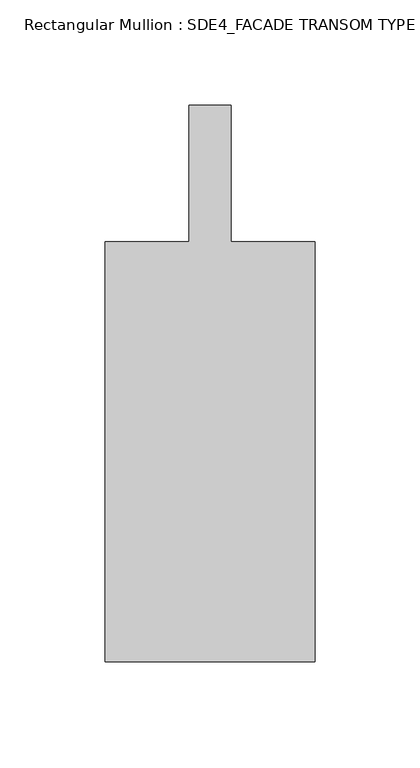
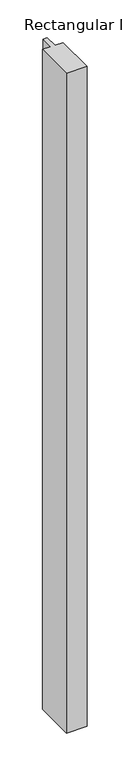
"""IFC4 building model written with IfcOpenShell, lengths in millimetres: member geometry, Rectangular Mullion : SDE4_FACADE TRANSOM TYPE 2."""

from ifc_helpers import new_model, si_unit, frame, origin, place, context, project, spatial, polyline, outline, extrude, source, transform, mapped, element, save


def rectangular_mullion_sde4_facade_transom_type_2_80bdb48c(model_context):
    return source(origin(), model_context, "Body", "SweptSolid", [
        extrude(outline(polyline([(50.0, -132.5), (-50.0, -132.5), (-50.0, 67.5), (-10.0, 67.5), (-10.0, 132.5), (10.0, 132.5), (10.0, 67.5), (50.0, 67.5), (50.0, -132.5)])), frame((0.0, 0.0, -3377.0), z_axis=(0.0, 0.0, 1.0), x_axis=(1.0, 0.0, 0.0)), (0.0, 0.0, 1.0), 3377.0),
    ])


if __name__ == "__main__":
    model = new_model("IFC4")
    model_context = context("Model", 3, world=origin())
    ifc_project = project(units=[si_unit("LENGTHUNIT", "METRE", prefix="MILLI")], contexts=[model_context])
    site = spatial("IfcSite", under=ifc_project)
    building = spatial("IfcBuilding", under=site)
    placement = place(None, origin())
    rectangular_mullion_sde4_facade_transom_type_2_shape = rectangular_mullion_sde4_facade_transom_type_2_80bdb48c(model_context)
    element("IfcMember", 1, ObjectType="Rectangular Mullion : SDE4_FACADE TRANSOM TYPE 2", at=placement, inside=building, context=model_context, shape_type="MappedRepresentation", body=[
        mapped(rectangular_mullion_sde4_facade_transom_type_2_shape, transform((0.0, 0.0, 0.0), x_axis=(1.0, 0.0, 0.0), y_axis=(0.0, 1.0, 0.0), z_axis=(0.0, 0.0, 1.0))),
    ])
    save(model, "model.ifc")

# Revit data of these elements
# Type "Rectangular Mullion : SDE4_FACADE TRANSOM TYPE 2"
#   built-in parameter 1007322 = 0.869423 (stored number, unit not read)
#   built-in parameter 1007321 = 0.164042 (stored number, unit not read)
#   built-in parameter 1007320 = 0.164042 (stored number, unit not read)
